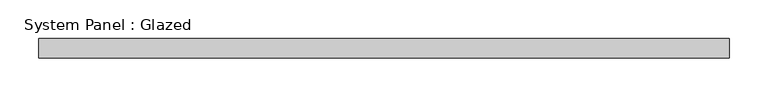
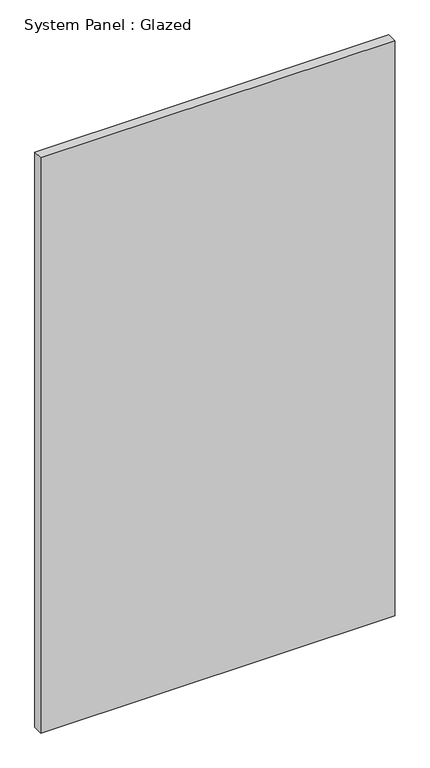
"""IFC4 building model written with IfcOpenShell, lengths in millimetres: plate geometry, System Panel : Glazed."""

from ifc_helpers import new_model, si_unit, origin, origin_with_axes, place, context, project, spatial, polyline, outline, extrude, source, transform, mapped, element, save


def system_panel_glazed_938e6c7f(model_context):
    return source(origin(), model_context, "Body", "SweptSolid", [
        extrude(outline(polyline([(443.75, 24.5), (-443.75, 24.5), (-443.75, 49.5), (443.75, 49.5), (443.75, 24.5)])), origin_with_axes(), (0.0, 0.0, 1.0), 1525.0),
    ])


if __name__ == "__main__":
    model = new_model("IFC4")
    model_context = context("Model", 3, world=origin())
    ifc_project = project(units=[si_unit("LENGTHUNIT", "METRE", prefix="MILLI")], contexts=[model_context])
    site = spatial("IfcSite", under=ifc_project)
    building = spatial("IfcBuilding", under=site)
    placement = place(None, origin())
    system_panel_glazed_shape = system_panel_glazed_938e6c7f(model_context)
    element("IfcPlate", 1, ObjectType="System Panel : Glazed", at=placement, inside=building, context=model_context, shape_type="MappedRepresentation", body=[
        mapped(system_panel_glazed_shape, transform((0.0, 0.0, 0.0), x_axis=(1.0, 0.0, 0.0), y_axis=(0.0, 1.0, 0.0), z_axis=(0.0, 0.0, 1.0))),
    ])
    save(model, "model.ifc")

# Revit data of these elements
# Type "System Panel : Glazed"
#   Construction Type Id = "GSP4R"
#   Analytic Construction = "1/8 in Pilkington single glazing"
#   Visual Light Transmittance = 0.9
#   Solar Heat Gain Coefficient = 0.86
#   Heat Transfer Coefficient (U) = 6.7069 W/(m²·K)
#   Define Thermal Properties by = 1
# Element 1 (IfcPlate, "System Panel : Glazed")
#   Materials on its faces: "Glass"
# Materials
#   "Glass": class "Glass", colour RGB 0 128 192, transparency 0.9, Description = "Soda Lime Glass", Cost = 0
